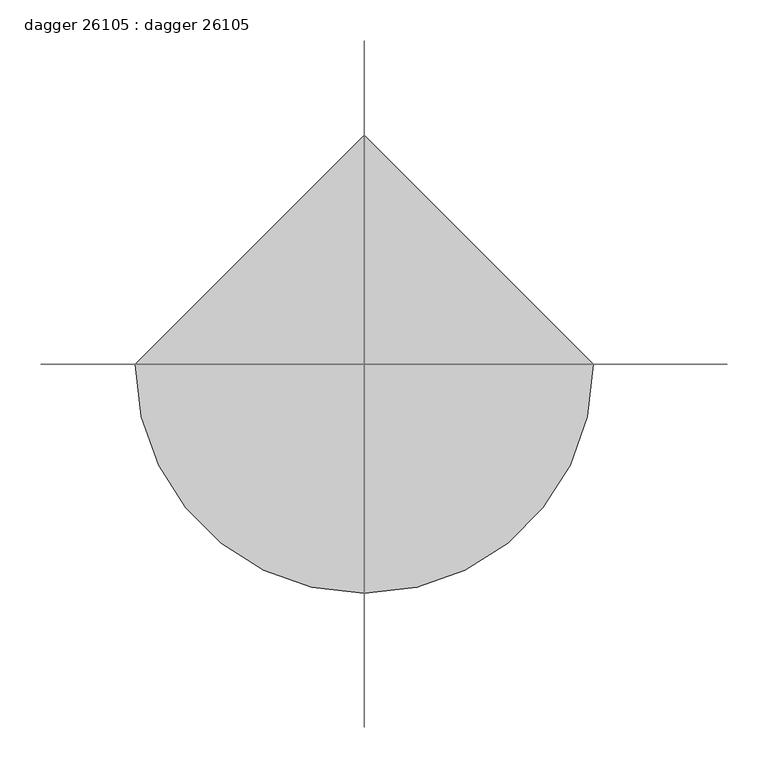
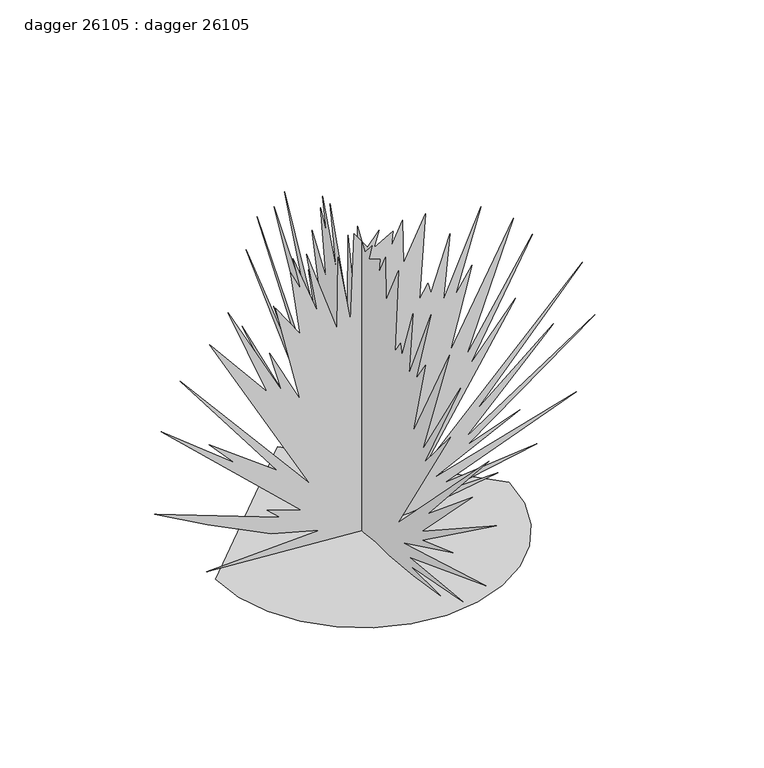
"""IFC4 building model written with IfcOpenShell, lengths in millimetres: proxy geometry, dagger 26105 : dagger 26105."""

from ifc_helpers import new_model, si_unit, origin, place, context, project, spatial, triangles, source, transform, mapped, element, save


def dagger_26105_dagger_26105_80c14bd7(model_context):
    return source(origin(), model_context, "Body", "Tessellation", [
        triangles([(-0.0169483, -5.816808, 0.0), (-0.0169288, 298.9836399, 21.1666745), (-0.0169413, 81.6722405, 29.6334406), (-0.0169342, 174.805482, 55.033464), (-0.0169232, 297.5713896, 117.1222841), (-0.0169138, 399.1714926, 173.5667131), (-0.0169336, 157.8723041, 83.2556831), (-0.0169307, 183.2723162, 105.8335019), (-0.016936, 116.9500744, 83.2556831), (-0.0169048, 386.4714684, 337.2563765), (-0.0169199, 245.3611499, 224.3667555), (-0.0169138, 294.7494507, 277.9879738), (-0.0169274, 163.5166906, 180.6223326), (-0.0169017, 349.7836641, 426.1564734), (-0.0169339, 101.427866, 132.6444926), (-0.0169017, 293.339762, 481.1881433), (-0.0169163, 183.2723162, 347.1344436), (-0.0169007, 258.0616646, 533.400436), (-0.0169184, 155.0501108, 340.0783336), (-0.0169121, 177.6279296, 423.3345162), (-0.0169223, 119.7722677, 309.0344436), (-0.0169075, 166.3388839, 510.8223447), (-0.0169144, 119.7722677, 443.088107), (-0.0169055, 138.1166785, 572.9127045), (-0.016909, 118.3610439, 533.400436), (-0.0169042, 132.4722829, 599.7224052), (-0.0169145, 85.9054123, 475.5442655), (-0.0169058, 107.0722617, 599.7224052), (-0.0169196, 47.8056303, 427.566162), (-0.016911, 46.3944065, 572.9127045), (-0.0169207, 22.4054592, 434.622272), (-0.0169106, 15.349867, 609.6005087), (-0.0169144, -10.050077, 572.9127045), (-0.0169141, -32.6278504, 599.7224052), (-0.0169154, -22.7501125, 567.2662831), (-0.0169164, -59.4390954, 588.4346495), (-0.0169179, -56.6168975, 560.2126802), (-0.0169166, -77.7834971, 603.9565945), (-0.0169218, -79.1947209, 516.4662226), (-0.0169192, -121.52792, 602.5443624), (-0.0169287, -110.2391378, 431.8003512), (-0.0169282, -127.17257, 458.6125955), (-0.0169297, -132.8169566, 437.4442291), (-0.0169255, -169.5057691, 544.6881918), (-0.0169325, -156.8057631, 414.8661378), (-0.0169271, -228.7723914, 578.5565824), (-0.0169337, -179.3835819, 417.6880949), (-0.0169328, -211.8392135, 465.6661983), (-0.0169399, -169.5057691, 304.8002543), (-0.0169334, -290.8607164, 533.400436), (-0.0169428, -200.550186, 286.4563522), (-0.0169383, -327.5510459, 488.2442533), (-0.0169445, -207.6057873, 265.2879677), (-0.0169435, -295.0948874, 369.7125349), (-0.0169498, -120.1169505, 88.9000696), (-0.0169494, -423.5072528, 397.9345041), (-0.016951, -218.8948329, 167.9223265), (-0.0169525, -368.473003, 292.1002301), (-0.0169526, -199.1392074, 119.9444865), (-0.0169578, -447.4950328, 282.222163), (-0.0169538, -201.9614007, 103.0113086), (-0.0169577, -303.5607224, 139.700112), (-0.0169526, -137.0501284, 59.2666313), (-0.0169642, -412.2169172, 138.2888882), (-0.0169548, -158.2169778, 42.3334534), (-0.0169644, -336.0168809, 59.2666313), (-0.0169559, -159.6279563, 25.4000212), (-0.0169619, -261.2290403, 26.811245), (-0.0169573, -170.9169838, 12.7000106), (-0.0169529, -89.0722793, 4.2333197), (-0.0169503, -43.9168869, 4.2333197), (-282.2577168, 0.0, 0.0937388), (-274.7951999, -64.6747996, 0.0937388), (-253.5445348, -124.0684354, 0.0937388), (-220.2049637, -176.4790898, 0.0937388), (-176.4790898, -220.2049637, 0.0937388), (-124.0684354, -253.5445348, 0.0937388), (-64.6747996, -274.7951999, 0.0937388), (1.23e-05, -282.2577168, 0.0937388), (64.6747996, -274.7951999, 0.0937388), (124.0684354, -253.5445348, 0.0937388), (176.4790898, -220.2049637, 0.0937388), (220.2049637, -176.4790898, 0.0937388), (253.5445348, -124.0684354, 0.0937388), (274.7951999, -64.6747996, 0.0937388), (282.2577168, 2.47e-05, 0.0937388), (-3.7e-05, 282.2577168, 0.0937388), (5.816808, 0.0169479, 0.0), (-298.9836399, 0.0169466, 21.1666745), (-81.6722405, 0.0169461, 29.6334406), (-174.8057363, 0.0169446, 55.033464), (-297.5713896, 0.0169409, 117.1222841), (-399.1714926, 0.0169375, 173.5667131), (-157.8723041, 0.016943, 83.2556831), (-183.2723162, 0.0169416, 105.8335019), (-116.9500744, 0.016943, 83.2556831), (-386.4714684, 0.0169278, 337.2563765), (-245.3611499, 0.0169345, 224.3667555), (-294.7494507, 0.0169313, 277.9879738), (-163.5166906, 0.0169371, 180.6223326), (-349.7836641, 0.0169225, 426.1564734), (-101.427866, 0.01694, 132.6444926), (-293.339762, 0.0169192, 481.1881433), (-183.2723162, 0.0169272, 347.1344436), (-258.0616646, 0.0169161, 533.400436), (-155.0501108, 0.0169277, 340.0783336), (-177.6279296, 0.0169227, 423.3345162), (-119.7722677, 0.0169295, 309.0344436), (-166.3388839, 0.0169175, 510.8223447), (-119.7722677, 0.0169215, 443.088107), (-138.1166785, 0.0169138, 572.9127045), (-118.3610439, 0.0169161, 533.400436), (-132.4722829, 0.0169121, 599.7224052), (-85.9054123, 0.0169196, 475.5442655), (-107.0722617, 0.0169121, 599.7224052), (-47.8056303, 0.0169224, 427.566162), (-46.3944065, 0.0169138, 572.9127045), (-22.4054592, 0.016922, 434.622272), (-15.3498931, 0.0169116, 609.6005087), (10.0501019, 0.0169138, 572.9127045), (32.6278504, 0.0169121, 599.7224052), (22.7501125, 0.0169141, 567.2662831), (59.4390954, 0.0169129, 588.4346495), (56.6168975, 0.0169145, 560.2126802), (77.7834971, 0.0169119, 603.9565945), (79.1947209, 0.0169171, 516.4662226), (121.52792, 0.016912, 602.5443624), (110.2391378, 0.0169222, 431.8003512), (127.17257, 0.0169206, 458.6125955), (132.8169566, 0.0169218, 437.4442291), (169.5057691, 0.0169154, 544.6881918), (156.8057631, 0.0169232, 414.8661378), (228.7723914, 0.0169134, 578.5565824), (179.3835819, 0.016923, 417.6880949), (211.8392135, 0.0169201, 465.6661983), (169.5057691, 0.0169297, 304.8002543), (290.8607164, 0.0169161, 533.400436), (200.550186, 0.0169308, 286.4563522), (327.5510459, 0.0169188, 488.2442533), (207.6057873, 0.0169321, 265.2879677), (295.0948874, 0.0169259, 369.7125349), (120.1169505, 0.0169426, 88.9000696), (423.5072528, 0.0169242, 397.9345041), (218.8948329, 0.0169379, 167.9223265), (368.473003, 0.0169305, 292.1002301), (199.1392074, 0.0169408, 119.9444865), (447.4950328, 0.0169311, 282.222163), (201.9614007, 0.0169418, 103.0113086), (303.5607224, 0.0169396, 139.700112), (137.0501284, 0.0169444, 59.2666313), (412.2169172, 0.0169397, 138.2888882), (158.2169778, 0.0169454, 42.3334534), (336.0168809, 0.0169444, 59.2666313), (159.6279563, 0.0169464, 25.4000212), (261.2290403, 0.0169463, 26.811245), (170.9169838, 0.0169471, 12.7000106), (89.0722793, 0.0169477, 4.2333197), (43.9168869, 0.0169477, 4.2333197)], [[68, 67, 69], [69, 67, 70], [64, 63, 65], [62, 61, 63], [58, 57, 59], [56, 55, 57], [57, 55, 59], [52, 51, 53], [50, 49, 51], [48, 47, 49], [46, 45, 47], [47, 45, 49], [40, 39, 41], [36, 35, 37], [34, 33, 35], [28, 27, 29], [26, 25, 27], [24, 23, 25], [22, 21, 23], [20, 19, 21], [16, 15, 17], [12, 11, 13], [10, 9, 11], [11, 9, 13], [8, 7, 9], [2, 1, 3], [66, 65, 67], [67, 65, 70], [65, 63, 70], [60, 59, 61], [61, 59, 63], [59, 55, 63], [63, 55, 70], [54, 53, 55], [53, 51, 55], [51, 49, 55], [49, 45, 55], [44, 43, 45], [45, 43, 55], [43, 42, 55], [42, 41, 55], [55, 41, 70], [41, 39, 70], [70, 39, 71], [39, 38, 71], [38, 37, 71], [37, 35, 71], [71, 35, 1], [35, 33, 1], [33, 32, 1], [18, 17, 19], [17, 15, 19], [19, 15, 21], [14, 13, 15], [13, 9, 15], [6, 5, 7], [5, 4, 7], [4, 3, 7], [7, 3, 9], [9, 3, 15], [21, 15, 23], [23, 15, 25], [25, 15, 27], [15, 3, 27], [27, 3, 29], [3, 1, 29], [29, 1, 30], [30, 1, 31], [1, 32, 31], [86, 87, 72], [85, 86, 72], [85, 72, 73], [84, 85, 73], [84, 73, 74], [84, 74, 75], [83, 84, 75], [82, 83, 75], [82, 75, 76], [82, 76, 77], [82, 77, 78], [82, 78, 79], [82, 79, 80], [82, 80, 81], [154, 155, 156], [154, 156, 157], [150, 151, 152], [148, 149, 150], [144, 145, 146], [142, 143, 144], [142, 144, 146], [138, 139, 140], [136, 137, 138], [134, 135, 136], [132, 133, 134], [132, 134, 136], [126, 127, 128], [122, 123, 124], [120, 121, 122], [114, 115, 116], [112, 113, 114], [110, 111, 112], [108, 109, 110], [106, 107, 108], [102, 103, 104], [98, 99, 100], [96, 97, 98], [96, 98, 100], [94, 95, 96], [88, 89, 90], [152, 153, 154], [152, 154, 157], [150, 152, 157], [146, 147, 148], [146, 148, 150], [142, 146, 150], [142, 150, 157], [140, 141, 142], [138, 140, 142], [136, 138, 142], [132, 136, 142], [130, 131, 132], [130, 132, 142], [129, 130, 142], [128, 129, 142], [128, 142, 157], [126, 128, 157], [126, 157, 158], [125, 126, 158], [124, 125, 158], [122, 124, 158], [122, 158, 88], [120, 122, 88], [119, 120, 88], [104, 105, 106], [102, 104, 106], [102, 106, 108], [100, 101, 102], [96, 100, 102], [92, 93, 94], [91, 92, 94], [90, 91, 94], [90, 94, 96], [90, 96, 102], [102, 108, 110], [102, 110, 112], [102, 112, 114], [90, 102, 114], [90, 114, 116], [88, 90, 116], [88, 116, 117], [88, 117, 118], [119, 88, 118]], closed=False),
    ])


if __name__ == "__main__":
    model = new_model("IFC4")
    model_context = context("Model", 3, world=origin())
    ifc_project = project(units=[si_unit("LENGTHUNIT", "METRE", prefix="MILLI")], contexts=[model_context])
    site = spatial("IfcSite", under=ifc_project)
    building = spatial("IfcBuilding", under=site)
    placement = place(None, origin())
    dagger_26105_dagger_26105_shape = dagger_26105_dagger_26105_80c14bd7(model_context)
    element("IfcBuildingElementProxy", 1, Name="dagger 26105 : dagger 26105", ObjectType="dagger 26105 : dagger 26105", at=placement, inside=building, context=model_context, shape_type="MappedRepresentation", body=[
        mapped(dagger_26105_dagger_26105_shape, transform((0.0, 0.0, 0.0), x_axis=(1.0, 0.0, 0.0), y_axis=(0.0, 1.0, 0.0), z_axis=(0.0, 0.0, 1.0))),
    ])
    save(model, "model.ifc")

# Revit data of these elements
# Type "dagger 26105 : dagger 26105"
#   built-in parameter 1005195 = "RPC-16-G3A7-NEG0-UH6H-J000-ST1L-LVER-AU"
#   Height = 0
